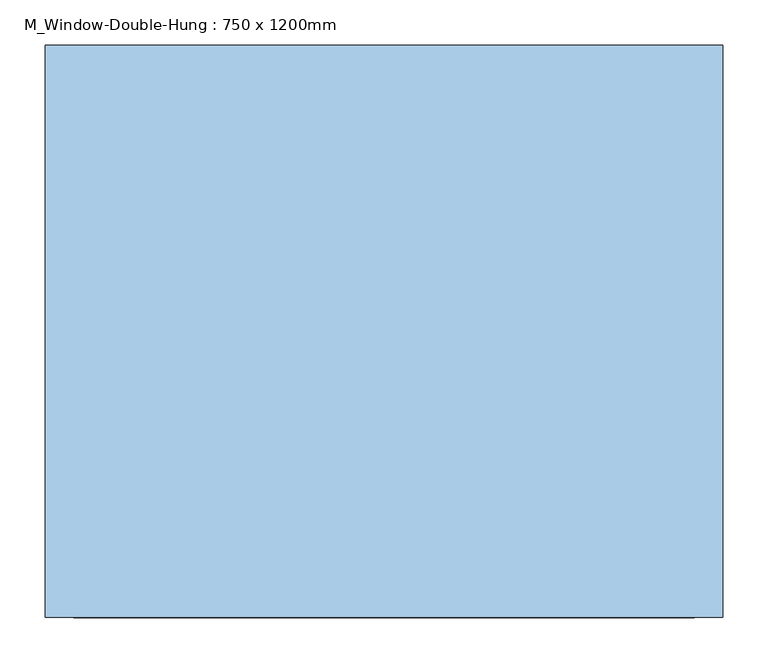
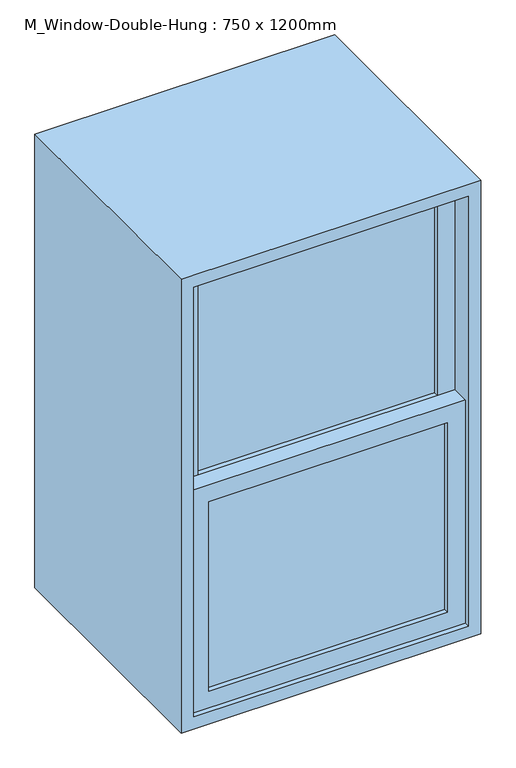
"""IFC4 building model written with IfcOpenShell, lengths in millimetres: window geometry, M_Window-Double-Hung : 750 x 1200mm."""

import ifcopenshell
import ifcopenshell.guid

model = None  # the IFC model being written
_history = None  # IfcOwnerHistory: only IFC2X3 demands one
_inside = {}  # id of a spatial element -> (the spatial element, [elements in it])
_under = {}  # id of a project, library or spatial element -> (it, [spatial elements below it])
_declared = {}  # id of a project -> (the project, [libraries it declares])
_typed = {}  # id of a type object -> (the type object, [elements of that type])
_made_of = {}  # id of a material, layer set ... -> (it, [elements and type objects made of it])


def new_model(schema):
    """Start an empty IFC model of exactly this schema.

    Asked for "IFC4X3", IfcOpenShell would pick the latest addendum, in which some entities
    have other attributes; the version numbers below select the first issue.
    IFC2X3 requires an IfcOwnerHistory on every rooted entity: one is made here for all.
    """
    global model, _history
    if schema == "IFC4X3":
        model = ifcopenshell.file(schema_version=(4, 3, 0, 0))
    else:
        model = ifcopenshell.file(schema=schema)
    _inside.clear()
    _under.clear()
    _declared.clear()
    _typed.clear()
    _made_of.clear()
    _history = None
    if model.schema == "IFC2X3":
        org = make("IfcOrganization", Name="unknown")
        user = make(
            "IfcPersonAndOrganization",
            ThePerson=make("IfcPerson", FamilyName="unknown"),
            TheOrganization=org,
        )
        app = make(
            "IfcApplication",
            ApplicationDeveloper=org,
            Version="unknown",
            ApplicationFullName="unknown",
            ApplicationIdentifier="unknown",
        )
        _history = make(
            "IfcOwnerHistory",
            OwningUser=user,
            OwningApplication=app,
            ChangeAction="ADDED",
            CreationDate=0,
        )
    return model


def make(cls, **values):
    """One entity of the class cls with the attributes given. An attribute that is None is left unset."""
    return model.create_entity(
        cls, **{name: value for name, value in values.items() if value is not None}
    )


def rooted(cls, **values):
    """An entity with a GlobalId (a new one), such as an element, a storey or a relation."""
    return make(cls, GlobalId=ifcopenshell.guid.new(), OwnerHistory=_history, **values)


def si_unit(unit_type, name, prefix=None):
    """IfcSIUnit, for example si_unit("LENGTHUNIT", "METRE", prefix="MILLI")."""
    return make("IfcSIUnit", UnitType=unit_type, Prefix=prefix, Name=name)


def assignment(units):
    """IfcUnitAssignment: the units of a project."""
    return None if units is None else make("IfcUnitAssignment", Units=units)


def point(xyz):
    """IfcCartesianPoint."""
    return None if xyz is None else make("IfcCartesianPoint", Coordinates=xyz)


def direction(xyz):
    """IfcDirection."""
    return None if xyz is None else make("IfcDirection", DirectionRatios=xyz)


def frame(location, z_axis=None, x_axis=None):
    """IfcAxis2Placement3D, a coordinate frame: its origin and axes. An axis left out is left unset."""
    return make(
        "IfcAxis2Placement3D",
        Location=point(location),
        Axis=direction(z_axis),
        RefDirection=direction(x_axis),
    )


def origin():
    """The frame at (0, 0, 0) with its axes left unset."""
    return frame((0.0, 0.0, 0.0))


def place(relative_to, where):
    """IfcLocalPlacement: puts the frame where relative to a parent placement (None: the world)."""
    return make(
        "IfcLocalPlacement", PlacementRelTo=relative_to, RelativePlacement=where
    )


def context(
    kind, dimensions, precision=None, world=None, true_north=None, identifier=None
):
    """IfcGeometricRepresentationContext, for example the 3D "Model" context."""
    return make(
        "IfcGeometricRepresentationContext",
        ContextIdentifier=identifier,
        ContextType=kind,
        CoordinateSpaceDimension=dimensions,
        Precision=precision,
        WorldCoordinateSystem=world,
        TrueNorth=true_north,
    )


def project(units=None, contexts=None):
    """IfcProject with its units and contexts."""
    return rooted(
        "IfcProject",
        Name="project",
        RepresentationContexts=contexts,
        UnitsInContext=assignment(units),
    )


def spatial(cls, under=None, at=None, **own):
    """A site, building, storey or space (cls), placed at a placement, below another one or the project."""
    s = rooted(cls, ObjectPlacement=at, **own)
    if under is not None:
        _under.setdefault(under.id(), (under, []))[1].append(s)
    return s


def polyline(points):
    """IfcPolyline through the points."""
    return make("IfcPolyline", Points=[point(p) for p in points])


def outline(outer, holes=None, kind="AREA"):
    """IfcArbitraryClosedProfileDef: a profile drawn as a closed curve; with holes, ...WithVoids."""
    if holes is None:
        return make("IfcArbitraryClosedProfileDef", ProfileType=kind, OuterCurve=outer)
    return make(
        "IfcArbitraryProfileDefWithVoids",
        ProfileType=kind,
        OuterCurve=outer,
        InnerCurves=holes,
    )


def extrude(swept, where, along, depth):
    """IfcExtrudedAreaSolid: the profile swept, set in the frame where, extruded along a direction by depth."""
    return make(
        "IfcExtrudedAreaSolid",
        SweptArea=swept,
        Position=where,
        ExtrudedDirection=direction(along),
        Depth=depth,
    )


def shape(context_of_items, identifier, shape_type, items):
    """IfcShapeRepresentation: the items that make up one representation, for example the "Body"."""
    return make(
        "IfcShapeRepresentation",
        ContextOfItems=context_of_items,
        RepresentationIdentifier=identifier,
        RepresentationType=shape_type,
        Items=items,
    )


def source(mapping_origin, context_of_items, identifier, shape_type, items):
    """IfcRepresentationMap: a shape defined once, which mapped items show again and again."""
    return make(
        "IfcRepresentationMap",
        MappingOrigin=mapping_origin,
        MappedRepresentation=shape(context_of_items, identifier, shape_type, items),
    )


def transform(
    local_origin,
    x_axis=None,
    y_axis=None,
    z_axis=None,
    scale=None,
    scale2=None,
    scale3=None,
    uniform=True,
):
    """IfcCartesianTransformationOperator3D, or its non-uniform kind. x_axis, y_axis, z_axis: its Axis1, 2, 3."""
    if uniform:
        return make(
            "IfcCartesianTransformationOperator3D",
            Axis1=direction(x_axis),
            Axis2=direction(y_axis),
            LocalOrigin=point(local_origin),
            Scale=scale,
            Axis3=direction(z_axis),
        )
    return make(
        "IfcCartesianTransformationOperator3DnonUniform",
        Axis1=direction(x_axis),
        Axis2=direction(y_axis),
        LocalOrigin=point(local_origin),
        Scale=scale,
        Axis3=direction(z_axis),
        Scale2=scale2,
        Scale3=scale3,
    )


def mapped(mapping_source, mapping_target):
    """IfcMappedItem: shows the shape of a source again, moved by a transform."""
    return make(
        "IfcMappedItem", MappingSource=mapping_source, MappingTarget=mapping_target
    )


def made_of(thing, what):
    """Note that an element or type object is made of a material, layer set ...; save() writes the relation."""
    if what is not None:
        _made_of.setdefault(what.id(), (what, []))[1].append(thing)
    return thing


def element(
    cls,
    number,
    at=None,
    inside=None,
    cuts=None,
    type_object=None,
    material=None,
    context=None,
    identifier="Body",
    shape_type=None,
    held_by="IfcProductDefinitionShape",
    body=None,
    shapes=None,
    **own,
):
    """One element of the class cls, such as IfcWall. Its Tag is "e" and its number.

    at: its placement. inside: the storey or other place that contains it. cuts: it is an
    opening in that element (IfcRelVoidsElement). A single representation is given by context,
    identifier, shape_type and body (its items); several are given by shapes. held_by: the class
    of the entity that holds the representations. save() writes the other relations.
    """
    e = rooted(cls, Tag="e%d" % number, ObjectPlacement=at, **own)
    if body is not None:
        shapes = [shape(context, identifier, shape_type, body)]
    if shapes is not None:
        e.Representation = make(held_by, Representations=shapes)
    if inside is not None:
        _inside.setdefault(inside.id(), (inside, []))[1].append(e)
    if cuts is not None:
        rooted(
            "IfcRelVoidsElement", RelatingBuildingElement=cuts, RelatedOpeningElement=e
        )
    if type_object is not None:
        _typed.setdefault(type_object.id(), (type_object, []))[1].append(e)
    return made_of(e, material)


def aggregate(whole, parts):
    """IfcRelAggregates: a whole, such as a stair, and the parts it consists of."""
    return rooted("IfcRelAggregates", RelatingObject=whole, RelatedObjects=parts)


def save(model, path):
    """Write the relations noted so far, then the file.

    IfcRelAggregates (storeys below a building ...), IfcRelContainedInSpatialStructure (elements
    in a storey), IfcRelDefinesByType, IfcRelAssociatesMaterial and IfcRelDeclares: one each for
    every whole, place, type object, material and project.
    """
    for whole, parts in _under.values():
        aggregate(whole, parts)
    for where, things in _inside.values():
        rooted(
            "IfcRelContainedInSpatialStructure",
            RelatedElements=things,
            RelatingStructure=where,
        )
    for kind, things in _typed.values():
        rooted("IfcRelDefinesByType", RelatedObjects=things, RelatingType=kind)
    for what, things in _made_of.values():
        rooted("IfcRelAssociatesMaterial", RelatedObjects=things, RelatingMaterial=what)
    for by, libraries in _declared.values():
        rooted("IfcRelDeclares", RelatingContext=by, RelatedDefinitions=libraries)
    model.write(path)


def m_window_double_hung_750_x_1200mm_e21ea802(model_context):
    return source(origin(), model_context, "Body", "SweptSolid", [
        extrude(outline(polyline([(298.8, -469.85), (298.8, -476.2), (-298.8, -476.2), (-298.8, -469.85), (298.8, -469.85)])), frame((0.0, 0.0, 990.6), z_axis=(0.0, 0.0, 1.0), x_axis=(1.0, 0.0, 0.0)), (0.0, 0.0, 1.0), 501.575),
        extrude(outline(polyline([(-298.8, -482.55), (298.8, -482.55), (298.8, -488.9), (-298.8, -488.9), (-298.8, -482.55)])), frame((0.0, 0.0, 990.6), z_axis=(0.0, 0.0, 1.0), x_axis=(1.0, 0.0, 0.0)), (0.0, 0.0, 1.0), 501.575),
        extrude(outline(polyline([(298.8, -425.4), (298.8, -431.75), (-298.8, -431.75), (-298.8, -425.4), (298.8, -425.4)])), frame((0.0, 0.0, 1536.625), z_axis=(0.0, 0.0, 1.0), x_axis=(1.0, 0.0, 0.0)), (0.0, 0.0, 1.0), 501.575),
        extrude(outline(polyline([(-298.8, -438.1), (298.8, -438.1), (298.8, -444.45), (-298.8, -444.45), (-298.8, -438.1)])), frame((0.0, 0.0, 1536.625), z_axis=(0.0, 0.0, 1.0), x_axis=(1.0, 0.0, 0.0)), (0.0, 0.0, 1.0), 501.575),
        extrude(outline(polyline([(1536.625, -343.25), (946.15, -343.25), (946.15, 343.25), (1536.625, 343.25), (1536.625, -343.25)]), holes=[polyline([(1492.175, 298.8), (990.6, 298.8), (990.6, -298.8), (1492.175, -298.8), (1492.175, 298.8)])]), frame((0.0, -501.6, 0.0), z_axis=(0.0, 1.0, 0.0), x_axis=(0.0, 0.0, 1.0)), (0.0, 0.0, 1.0), 44.45),
        extrude(outline(polyline([(2082.65, -343.25), (1492.175, -343.25), (1492.175, 343.25), (2082.65, 343.25), (2082.65, -343.25)]), holes=[polyline([(2038.2, 298.8), (1536.625, 298.8), (1536.625, -298.8), (2038.2, -298.8), (2038.2, 298.8)])]), frame((0.0, -457.15, 0.0), z_axis=(0.0, 1.0, 0.0), x_axis=(0.0, 0.0, 1.0)), (0.0, 0.0, 1.0), 44.45),
        extrude(outline(polyline([(2114.4, -375.0), (914.4, -375.0), (914.4, 375.0), (2114.4, 375.0), (2114.4, -375.0)]), holes=[polyline([(2082.65, 343.25), (946.15, 343.25), (946.15, -343.25), (2082.65, -343.25), (2082.65, 343.25)])]), frame((0.0, -514.3, 0.0), z_axis=(0.0, 1.0, 0.0), x_axis=(0.0, 0.0, 1.0)), (0.0, 0.0, 1.0), 633.35),
    ])


if __name__ == "__main__":
    model = new_model("IFC4")
    model_context = context("Model", 3, world=origin())
    ifc_project = project(units=[si_unit("LENGTHUNIT", "METRE", prefix="MILLI")], contexts=[model_context])
    site = spatial("IfcSite", under=ifc_project)
    building = spatial("IfcBuilding", under=site)
    placement = place(None, origin())
    m_window_double_hung_750_x_1200mm_shape = m_window_double_hung_750_x_1200mm_e21ea802(model_context)
    element("IfcWindow", 1, ObjectType="M_Window-Double-Hung : 750 x 1200mm", at=placement, inside=building, context=model_context, shape_type="MappedRepresentation", body=[
        mapped(m_window_double_hung_750_x_1200mm_shape, transform((0.0, 0.0, 0.0), x_axis=(1.0, 0.0, 0.0), y_axis=(0.0, 1.0, 0.0), z_axis=(0.0, 0.0, 1.0))),
    ])
    save(model, "model.ifc")

# Revit data of these elements
# Type "M_Window-Double-Hung : 750 x 1200mm"
#   Type Mark = "22"
#   Fire Rating = "0.5h"
#   Construction Type Id = "DG-DR"
#   Assembly Code = "B2020100"
#   Analytic Construction = "Double glazing - domestic"
#   Wall Thickness [instance default] = 150 mm
#   Window Inset [instance default] = 0 mm
#   Visual Light Transmittance = 0.81
#   Thermal Resistance (R) = 0.319569 (m²·K)/W
#   Solar Heat Gain Coefficient = 0.76
#   Muntin Width = 597.6 mm
#   Muntin Height = 501.575 mm
#   Interior Wall Closure [instance default] = 35.7 mm
#   Rough Width = 765 mm
#   Rough Height = 1215 mm
#   Frame Extension [instance default] = 31.75 mm
#   Exterior Wall Closure [instance default] = 12.7 mm
#   Extension Jamb [instance default] = 35.7 mm
#   Heat Transfer Coefficient (U) = 3.12929 W/(m²·K)
#   Height = 1200 mm
#   Width = 750 mm
#   Define Thermal Properties by = 1
#   Top Muntin Visibility = yes
#   Indicator Visibility [instance default] = yes
#   Extension Jamb Visibility [instance default] = yes
#   Interior Trim Visibility [instance default] = yes
#   Exterior Trim Visibility [instance default] = yes
#   Define Thermal Properties by = 1
#   Bottom Muntin Visibility = yes
#   Muntin Pattern = M_Muntin Pattern_2x2 : M_Muntin Pattern_2x2
#   Interior Trim Material = Wood - Stained
#   Interior Trim = M_Trim-Window-Interior-Flat : Picture Frame
#   Exterior Trim Material = Clad - White
#   Exterior Trim = M_Trim-Window-Exterior-Flat : with Sill
#   Glass Panel Material = Glass
#   Exterior Frame Material = Clad - White
#   Interior Frame Material = Wood - Stained
#   Wall Closure = (empty or 0)
# Element 1 (IfcWindow, "M_Window-Double-Hung : 750 x 1200mm")
#   Wall Thickness = 200 mm
#   Window Inset = 500 mm
#   Frame Extension = 531.75 mm
#   Extension Jamb = 25.4 mm
#   Extension Jamb Visibility = no
#   Materials on its faces: "Wood - Stained", "Glass", "Clad - White"
# Materials
#   "Wood - Stained": class "Wood", colour RGB 224 178 126, transparency 0, Cost = 0
#   "Clad - White": class "Wood", colour RGB 242 242 238, transparency 0, Cost = 0
#   "Glass": class "Glass", colour RGB 0 128 192, transparency 0.9, Description = "Soda Lime Glass", Cost = 0
